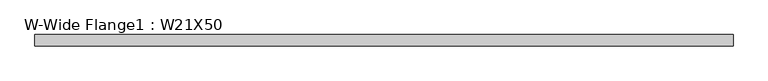
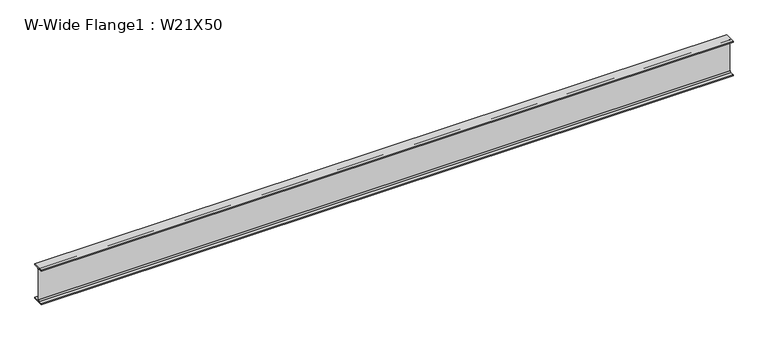
"""IFC4 building model written with IfcOpenShell, lengths in millimetres: beam geometry, W-Wide Flange1 : W21X50."""

from ifc_helpers import new_model, si_unit, point, frame, frame_2d, origin, place, context, project, spatial, polyline, circle_curve, trimmed, segment, composite_curve, outline, extrude, source, transform, mapped, element, save


def w_wide_flange1_w21x50_b5c1cd8e(model_context):
    return source(origin(), model_context, "Body", "SweptSolid", [
        extrude(outline(composite_curve([segment(polyline([(82.931, -250.571), (82.931, -264.16), (-82.931, -264.16), (-82.931, -250.571), (-22.987, -250.571)]), True, "CONTINUOUS"), segment(trimmed(circle_curve(frame_2d((-22.987, -232.41)), 18.161), [point((-22.987, -250.571))], [point((-4.826, -232.41))], True, "CARTESIAN"), True, "CONTINUOUS"), segment(polyline([(-4.826, -232.41), (-4.826, 232.41)]), True, "CONTINUOUS"), segment(trimmed(circle_curve(frame_2d((-22.987, 232.41)), 18.161), [point((-4.826, 232.41))], [point((-22.987, 250.571))], True, "CARTESIAN"), True, "CONTINUOUS"), segment(polyline([(-22.987, 250.571), (-82.931, 250.571), (-82.931, 264.16), (82.931, 264.16), (82.931, 250.571), (22.987, 250.571)]), True, "CONTINUOUS"), segment(trimmed(circle_curve(frame_2d((22.987, 232.41)), 18.161), [point((22.987, 250.571))], [point((4.826, 232.41))], True, "CARTESIAN"), True, "CONTINUOUS"), segment(polyline([(4.826, 232.41), (4.826, -232.41)]), True, "CONTINUOUS"), segment(trimmed(circle_curve(frame_2d((22.987, -232.41)), 18.161), [point((4.826, -232.41))], [point((22.987, -250.571))], True, "CARTESIAN"), True, "CONTINUOUS"), segment(polyline([(22.987, -250.571), (82.931, -250.571)]), True, "CONTINUOUS")], self_intersect=False)), frame((-5032.8483619, 0.0, 0.0), z_axis=(1.0, 0.0, 0.0), x_axis=(0.0, 1.0, 0.0)), (0.0, 0.0, 1.0), 10065.6967239),
    ])


if __name__ == "__main__":
    model = new_model("IFC4")
    model_context = context("Model", 3, world=origin())
    ifc_project = project(units=[si_unit("LENGTHUNIT", "METRE", prefix="MILLI")], contexts=[model_context])
    site = spatial("IfcSite", under=ifc_project)
    building = spatial("IfcBuilding", under=site)
    placement = place(None, origin())
    w_wide_flange1_w21x50_shape = w_wide_flange1_w21x50_b5c1cd8e(model_context)
    element("IfcBeam", 1, ObjectType="W-Wide Flange1 : W21X50", at=placement, inside=building, context=model_context, shape_type="MappedRepresentation", body=[
        mapped(w_wide_flange1_w21x50_shape, transform((0.0, 0.0, 0.0), x_axis=(1.0, 0.0, 0.0), y_axis=(0.0, 1.0, 0.0), z_axis=(0.0, 0.0, 1.0))),
    ])
    save(model, "model.ifc")

# Revit data of these elements
# Type "W-Wide Flange1 : W21X50"
#   Assembly Code = "B10"
#   W = 50
#   Start Extension Calculation [instance default] = 10' - 0"
#   Start Extension [instance default] = -0' - 0 1/2"
#   End Extension Calculation [instance default] = 10' - 0"
#   End Extension [instance default] = -0' - 0 1/2"
#   Length [instance default] = 5' - 0"
#   bf = 0' - 6.53"
#   d = 1' - 8.8"
#   k = 0' - 1 1/4"
#   k2 = 0' - 0.715"
#   tf = 0' - 0.535"
#   tw = 0' - 0.38"
#   A = 0.102083 SF
#   Structural Material [instance default] = Metal - Steel - ASTM A992
# Element 1 (IfcBeam, "W-Wide Flange1 : W21X50")
#   Materials on its faces: "Metal - Steel - ASTM A992"
# Materials
#   "Metal - Steel - ASTM A992": class "Metal", colour RGB 199 199 199, transparency 0
